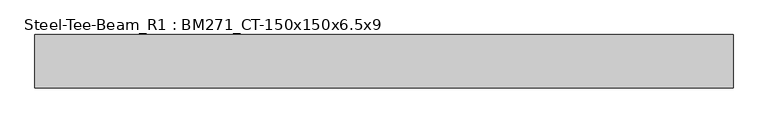
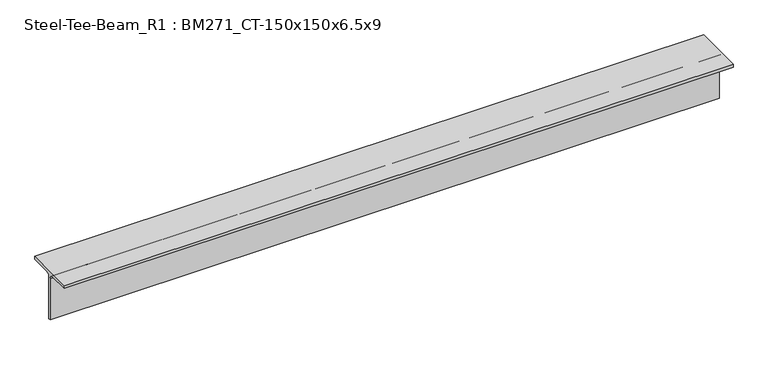
"""IFC4 building model written with IfcOpenShell, lengths in millimetres: member geometry, Steel-Tee-Beam_R1 : BM271_CT-150x150x6.5x9."""

from ifc_helpers import new_model, si_unit, point, frame, frame_2d, origin, place, context, project, spatial, polyline, circle_curve, trimmed, segment, composite_curve, outline, extrude, source, transform, mapped, element, save


def steel_tee_beam_r1_bm271_ct_150x150x6_5x9_cf272016(model_context):
    return source(origin(), model_context, "Body", "SweptSolid", [
        extrude(outline(composite_curve([segment(polyline([(75.0, 75.0), (75.0, 66.0), (16.25, 66.0)]), True, "CONTINUOUS"), segment(trimmed(circle_curve(frame_2d((16.25, 53.0)), 13.0), [point((16.25, 66.0))], [point((3.25, 53.0))], True, "CARTESIAN"), True, "CONTINUOUS"), segment(polyline([(3.25, 53.0), (3.25, -75.0), (-3.25, -75.0), (-3.25, 53.0)]), True, "CONTINUOUS"), segment(trimmed(circle_curve(frame_2d((-16.25, 53.0)), 13.0), [point((-3.25, 53.0))], [point((-16.25, 66.0))], True, "CARTESIAN"), True, "CONTINUOUS"), segment(polyline([(-16.25, 66.0), (-75.0, 66.0), (-75.0, 75.0), (75.0, 75.0)]), True, "CONTINUOUS")], self_intersect=False)), frame((-983.9814396, 0.0, 0.0), z_axis=(1.0, 0.0, 0.0), x_axis=(0.0, 1.0, 0.0)), (0.0, 0.0, 1.0), 1967.9628792),
    ])


if __name__ == "__main__":
    model = new_model("IFC4")
    model_context = context("Model", 3, world=origin())
    ifc_project = project(units=[si_unit("LENGTHUNIT", "METRE", prefix="MILLI")], contexts=[model_context])
    site = spatial("IfcSite", under=ifc_project)
    building = spatial("IfcBuilding", under=site)
    placement = place(None, origin())
    steel_tee_beam_r1_bm271_ct_150x150x6_5x9_shape = steel_tee_beam_r1_bm271_ct_150x150x6_5x9_cf272016(model_context)
    element("IfcMember", 1, ObjectType="Steel-Tee-Beam_R1 : BM271_CT-150x150x6.5x9", at=placement, inside=building, context=model_context, shape_type="MappedRepresentation", body=[
        mapped(steel_tee_beam_r1_bm271_ct_150x150x6_5x9_shape, transform((0.0, 0.0, 0.0), x_axis=(1.0, 0.0, 0.0), y_axis=(0.0, 1.0, 0.0), z_axis=(0.0, 0.0, 1.0))),
    ])
    save(model, "model.ifc")

# Revit data of these elements
# Type "Steel-Tee-Beam_R1 : BM271_CT-150x150x6.5x9"
#   Keynote = "CT-150x150x6.5x9"
#   Surface Area = 0.588841 m²/m
#   Section Area = 23.3904 cm²
#   Mass per Unit Length = 18.3614 kg/m
#   Length [instance default] = 1.5240 m
#   bf = 0.1500 m
#   d = 0.1500 m
#   k = 0.0220 m
#   r = 0.0130 m
#   tf = 0.0090 m
#   tw = 0.0065 m
#   hec_material4 [instance default] = none
#   hec_material3 [instance default] = none
#   hec_material2 [instance default] = none
#   hec_material1 [instance default] = none
#   Structural Material [instance default] = Steel, 45-345
#   Assembly Code = ""
# Element 1 (IfcMember, "Steel-Tee-Beam_R1 : BM271_CT-150x150x6.5x9")
#   Structural Material = none
# Materials
#   "Steel, 45-345": class "Metal", colour RGB 189 187 185, transparency 0, Description = "Steel 345 MPa", Cost = 0
